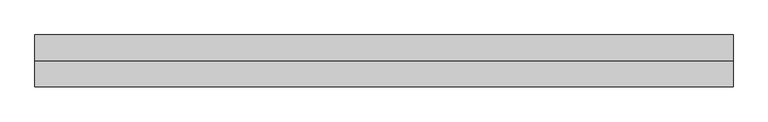
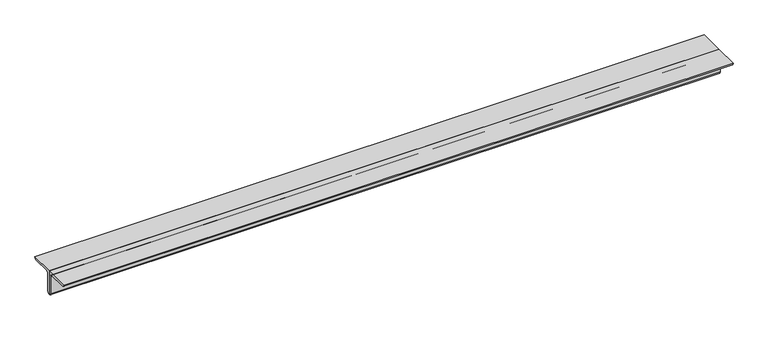
"""IFC4 building model written with IfcOpenShell, lengths in millimetres: beam geometry, 0123_Steel Framing_2Ls-KSD3502 : H_SB_AR_S04_2Ls-130x130x12_VBR1."""

from ifc_helpers import new_model, si_unit, point, frame, frame_2d, origin, place, context, project, spatial, polyline, circle_curve, trimmed, segment, composite_curve, outline, extrude, source, transform, mapped, element, save


def beam_96e87236(model_context):
    return source(origin(), model_context, "Body", "SweptSolid", [
        extrude(outline(composite_curve([segment(polyline([(0.0, 36.4), (130.0, 36.4)]), True, "CONTINUOUS"), segment(trimmed(circle_curve(frame_2d((118.0, 36.4)), 12.0), [point((130.0, 36.4))], [point((118.0, 24.4))], False, "CARTESIAN"), True, "CONTINUOUS"), segment(polyline([(118.0, 24.4), (24.0, 24.4)]), True, "CONTINUOUS"), segment(trimmed(circle_curve(frame_2d((24.0, 12.4)), 12.0), [point((24.0, 24.4))], [point((12.0, 12.4))], True, "CARTESIAN"), True, "CONTINUOUS"), segment(polyline([(12.0, 12.4), (12.0, -81.6)]), True, "CONTINUOUS"), segment(trimmed(circle_curve(frame_2d((0.0, -81.6)), 12.0), [point((12.0, -81.6))], [point((0.0, -93.6))], False, "CARTESIAN"), True, "CONTINUOUS"), segment(polyline([(0.0, -93.6), (0.0, 36.4)]), True, "CONTINUOUS")], self_intersect=False)), frame((-1749.149537, 0.0, 0.0), z_axis=(1.0, 0.0, 0.0), x_axis=(0.0, 1.0, 0.0)), (0.0, 0.0, 1.0), 3498.299074),
        extrude(outline(composite_curve([segment(polyline([(0.0, 36.4), (0.0, -93.6)]), True, "CONTINUOUS"), segment(trimmed(circle_curve(frame_2d((0.0, -81.6)), 12.0), [point((0.0, -93.6))], [point((-12.0, -81.6))], False, "CARTESIAN"), True, "CONTINUOUS"), segment(polyline([(-12.0, -81.6), (-12.0, 12.4)]), True, "CONTINUOUS"), segment(trimmed(circle_curve(frame_2d((-24.0, 12.4)), 12.0), [point((-12.0, 12.4))], [point((-24.0, 24.4))], True, "CARTESIAN"), True, "CONTINUOUS"), segment(polyline([(-24.0, 24.4), (-118.0, 24.4)]), True, "CONTINUOUS"), segment(trimmed(circle_curve(frame_2d((-118.0, 36.4)), 12.0), [point((-118.0, 24.4))], [point((-130.0, 36.4))], False, "CARTESIAN"), True, "CONTINUOUS"), segment(polyline([(-130.0, 36.4), (0.0, 36.4)]), True, "CONTINUOUS")], self_intersect=False)), frame((-1749.149537, 0.0, 0.0), z_axis=(1.0, 0.0, 0.0), x_axis=(0.0, 1.0, 0.0)), (0.0, 0.0, 1.0), 3498.299074),
    ])


if __name__ == "__main__":
    model = new_model("IFC4")
    model_context = context("Model", 3, world=origin())
    ifc_project = project(units=[si_unit("LENGTHUNIT", "METRE", prefix="MILLI")], contexts=[model_context])
    site = spatial("IfcSite", under=ifc_project)
    building = spatial("IfcBuilding", under=site)
    placement = place(None, origin())
    beam_shape = beam_96e87236(model_context)
    element("IfcBeam", 1, ObjectType="0123_Steel Framing_2Ls-KSD3502 : H_SB_AR_S04_2Ls-130x130x12_VBR1", at=placement, inside=building, context=model_context, shape_type="MappedRepresentation", body=[
        mapped(beam_shape, transform((0.0, 0.0, 0.0), x_axis=(1.0, 0.0, 0.0), y_axis=(0.0, 1.0, 0.0), z_axis=(0.0, 0.0, 1.0))),
    ])
    save(model, "model.ifc")

# Revit data of these elements
# Type "0123_Steel Framing_2Ls-KSD3502 : H_SB_AR_S04_2Ls-130x130x12_VBR1"
#   Type Mark = "VBR1"
#   Assembly Code = "B10"
#   Legs = "SLBB"
#   W = 8.97
#   Perimeter = 1.04 m²/m
#   Nominal Weight = 46.80 kgf/m
#   Length [instance default] = 1000 mm
#   Space = 0 mm
#   b = 130 mm
#   d = 130 mm
#   t = 12 mm
#   y = 36.4 mm
#   A = 0.005952 m²
#   Structural Material [instance default] = Steel ASTM A36
# Element 1 (IfcBeam, "0123_Steel Framing_2Ls-KSD3502 : H_SB_AR_S04_2Ls-130x130x12_VBR1")
#   Materials on its faces: "Steel ASTM A36"
# Materials
#   "Steel ASTM A36": class "Metal", colour RGB 199 199 199, transparency 0, Description = "Structural steel, ASTM A36 Grade B, mill finish", Cost = 0
